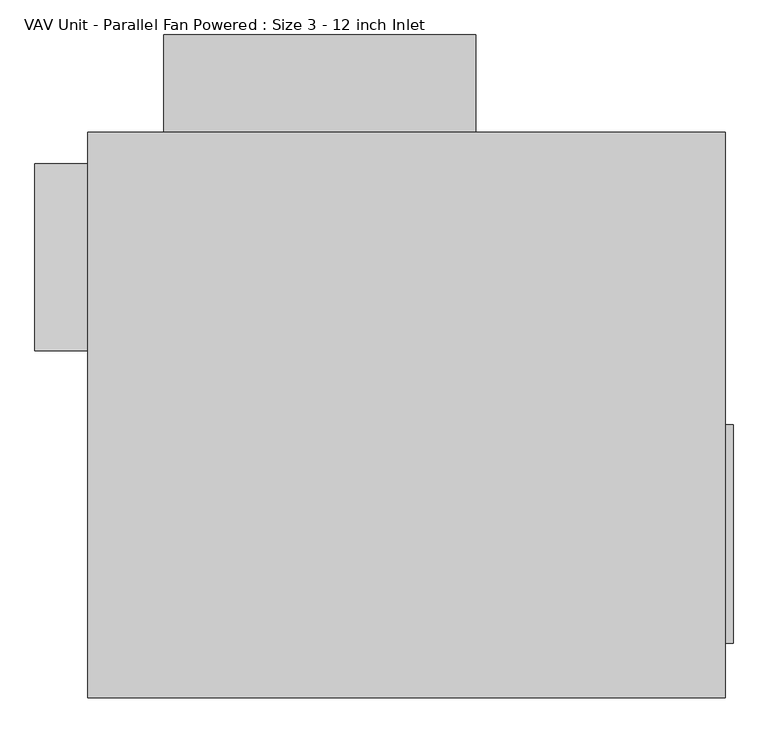
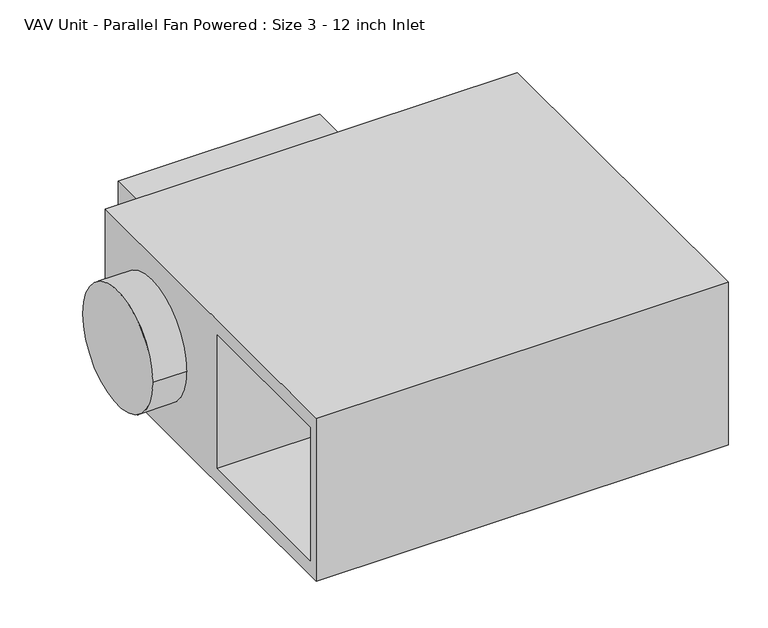
"""IFC4 building model written with IfcOpenShell, lengths in millimetres: proxy geometry, VAV Unit - Parallel Fan Powered : Size 3 - 12 inch Inlet."""

from ifc_helpers import new_model, si_unit, point, frame, frame_2d, origin, place, context, project, spatial, polyline, circle_curve, trimmed, segment, composite_curve, outline, extrude, faceted_brep, source, transform, mapped, element, save


def vav_unit_parallel_fan_powered_size_3_12_inch_inlet_966b65e1(model_context):
    return source(origin(), model_context, "Body", "SolidModel", [
        extrude(outline(polyline([(531.8125, -15.875), (531.8125, -371.475), (519.1125, -371.475), (519.1125, -15.875), (531.8125, -15.875)])), frame((0.0, 0.0, -139.7), z_axis=(0.0, 0.0, 1.0), x_axis=(1.0, 0.0, 0.0)), (0.0, 0.0, 1.0), 279.4),
        extrude(outline(polyline([(112.7125, 460.375), (-395.2875, 460.375), (-395.2875, 619.125), (112.7125, 619.125), (112.7125, 460.375)])), frame((0.0, 0.0, -152.4), z_axis=(0.0, 0.0, 1.0), x_axis=(1.0, 0.0, 0.0)), (0.0, 0.0, 1.0), 304.8),
        extrude(outline(composite_curve([segment(trimmed(circle_curve(frame_2d((257.175, 0.0)), 152.4), [point((104.775, 0.0))], [point((409.575, 0.0))], False, "CARTESIAN"), True, "CONTINUOUS"), segment(trimmed(circle_curve(frame_2d((257.175, 0.0)), 152.4), [point((409.575, 0.0))], [point((104.775, 0.0))], False, "CARTESIAN"), True, "CONTINUOUS")], self_intersect=False)), frame((-604.8375, 0.0, 0.0), z_axis=(1.0, 0.0, 0.0), x_axis=(0.0, 1.0, 0.0)), (0.0, 0.0, 1.0), 85.725),
        faceted_brep([(519.1125, 460.375, 217.4875), (-519.1125, 460.375, 217.4875), (-519.1125, -460.375, 217.4875), (519.1125, -460.375, 217.4875), (519.1125, 460.375, -217.4875), (519.1125, -460.375, -217.4875), (-519.1125, -460.375, -217.4875), (-519.1125, 460.375, -217.4875), (-519.1125, -434.975, 177.8), (-519.1125, -434.975, -177.8), (-519.1125, -28.575, -177.8), (-519.1125, -28.575, 177.8), (0.0, -434.975, 177.8), (0.0, -28.575, 177.8), (0.0, -28.575, -177.8), (0.0, -434.975, -177.8)], [[[0, 1, 2, 3]], [[4, 5, 6, 7]], [[1, 0, 4, 7]], [[2, 1, 7, 6], [8, 9, 10, 11]], [[3, 2, 6, 5]], [[0, 3, 5, 4]], [[12, 13, 14, 15]], [[12, 15, 9, 8]], [[15, 14, 10, 9]], [[14, 13, 11, 10]], [[13, 12, 8, 11]]]),
    ])


if __name__ == "__main__":
    model = new_model("IFC4")
    model_context = context("Model", 3, world=origin())
    ifc_project = project(units=[si_unit("LENGTHUNIT", "METRE", prefix="MILLI")], contexts=[model_context])
    site = spatial("IfcSite", under=ifc_project)
    building = spatial("IfcBuilding", under=site)
    placement = place(None, origin())
    vav_unit_parallel_fan_powered_size_3_12_inch_inlet_shape = vav_unit_parallel_fan_powered_size_3_12_inch_inlet_966b65e1(model_context)
    element("IfcBuildingElementProxy", 1, Name="VAV Unit - Parallel Fan Powered : Size 3 - 12 inch Inlet", ObjectType="VAV Unit - Parallel Fan Powered : Size 3 - 12 inch Inlet", at=placement, inside=building, context=model_context, shape_type="MappedRepresentation", body=[
        mapped(vav_unit_parallel_fan_powered_size_3_12_inch_inlet_shape, transform((0.0, 0.0, 0.0), x_axis=(1.0, 0.0, 0.0), y_axis=(0.0, 1.0, 0.0), z_axis=(0.0, 0.0, 1.0))),
    ])
    save(model, "model.ifc")

# Revit data of these elements
# Project information
#   Project Issue Date = "Issue Date"
#   Project Status = "Project Status"
#   Client Name = "Owner"
#   Project Address = "Enter address here"
#   Project Name = "Project Name"
#   Project Number = "Project Number"
# Type "VAV Unit - Parallel Fan Powered : Size 3 - 12 inch Inlet"
#   Width2 = 1' - 2"
#   Voltage = 120 V
#   UnitWidth = 3' - 4 7/8"
#   UnitHeight = 3' - 0 1/4"
#   UnitDepth = 1' - 5 1/8"
#   SupplyConnectorWidth = 1' - 2"
#   SupplyConnectorVerticalOffset = 0' - 2 1/8"
#   SupplyConnectorLength = 0' - 0 1/2"
#   SupplyConnectorHorizontalOffset = 0' - 3 1/2"
#   SupplyConnectorDepth = 0' - 11"
#   SupplyAirConnectorCenterOffset = 0' - 10 1/2"
#   PrimaryToSupplyRatio [instance default] = 0.2
#   PrimaryAirOffset = 0' - 8"
#   PrimaryAirFlow [instance default] = 400 CFM
#   PrimaryAirConnectorVerticalOffset = 0' - 8 9/16"
#   PrimaryAirConnectorRadius = 0' - 6"
#   PrimaryAirConnectorLength = 0' - 3 3/8"
#   PrimaryAirConnectorDiameter = 1' - 0"
#   PrimaryAirConnectorCenterOffset = 0' - 8"
#   Pressure Drop [instance default] = 0.01 in-wg
#   InducedAirInletWidth = 1' - 4"
#   InducedAirInletDepth = 1' - 2"
#   InducedAirConnectorHorizontalOffset = 0' - 1"
#   InducedAirConnectorCenterOffset = 0' - 9"
#   Height2 = 0' - 11"
#   ElectricalConnectionBoxWidth = 1' - 8"
#   ElectricalConnectionBoxOffset = 0' - 4 7/8"
#   ElectricalConnectionBoxHeight = 0' - 6 1/4"
#   ElectricalConnectionBoxDepth = 1' - 0"
#   SupplyAirFlow [instance default] = 2000 CFM
#   Apparent Load = 542 VA
#   SupplyAirConnectorIndex = 2
#   PrimaryAirConnectorIndex = 1
#   Number of Poles = 1
#   InducedAirConnectorIndex = 3
#   VAV Material = none
#   Load Classification = Cooling
#   Default Elevation = 0
#   Assembly Code = ""
